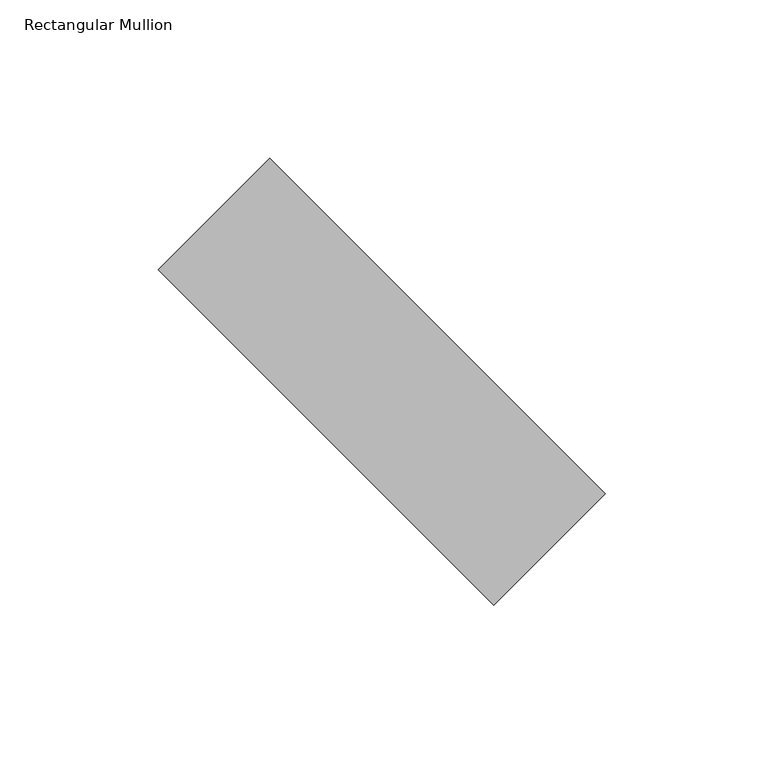
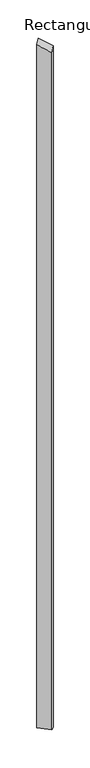
"""IFC4 building model written with IfcOpenShell, lengths in millimetres: member geometry, Rectangular Mullion : tilted mullions."""

from ifc_helpers import new_model, si_unit, origin, place, context, project, spatial, faceted_brep, source, transform, mapped, element, save


def rectangular_mullion_98a71f57(model_context):
    return source(origin(), model_context, "Body", "Brep", [
        faceted_brep([(-35.3553391, 70.7106781, -7999.3473161), (70.7106781, -35.3553391, -7999.3473161), (35.3553391, -70.7106781, -7999.3473161), (-70.7106781, 35.3553391, -7999.3473161), (-70.7106781, 35.3553391, 10.1224649), (-35.3553391, 70.7106781, 55.1417053), (35.3553391, -70.7106781, -55.1417053), (70.7106781, -35.3553391, -10.1224649)], [[[0, 1, 2, 3]], [[4, 5, 0, 3]], [[6, 4, 3, 2]], [[7, 6, 2, 1]], [[5, 7, 1, 0]], [[5, 4, 6, 7]]]),
    ])


if __name__ == "__main__":
    model = new_model("IFC4")
    model_context = context("Model", 3, world=origin())
    ifc_project = project(units=[si_unit("LENGTHUNIT", "METRE", prefix="MILLI")], contexts=[model_context])
    site = spatial("IfcSite", under=ifc_project)
    building = spatial("IfcBuilding", under=site)
    placement = place(None, origin())
    rectangular_mullion_shape = rectangular_mullion_98a71f57(model_context)
    element("IfcMember", 1, ObjectType="Rectangular Mullion : tilted mullions", at=placement, inside=building, context=model_context, shape_type="MappedRepresentation", body=[
        mapped(rectangular_mullion_shape, transform((0.0, 0.0, 0.0), x_axis=(1.0, 0.0, 0.0), y_axis=(0.0, 1.0, 0.0), z_axis=(0.0, 0.0, 1.0))),
    ])
    save(model, "model.ifc")

# Revit data of these elements
# Type "Rectangular Mullion : tilted mullions"
#   built-in parameter 1007304 = 0.492126 (stored number, unit not read)
#   built-in parameter 1007301 = 0.082021 (stored number, unit not read)
#   built-in parameter 1007300 = 0.082021 (stored number, unit not read)
# Element 1 (IfcMember, "Rectangular Mullion : tilted mullions")
#   Materials on its faces: "Aluminum"
# Materials
#   "Aluminum": class "Metal", colour RGB 244 244 244, transparency 0, Description = "Aluminum 6061", Cost = 0
